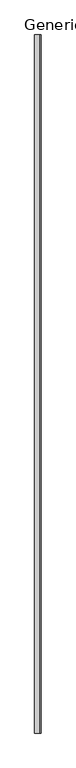
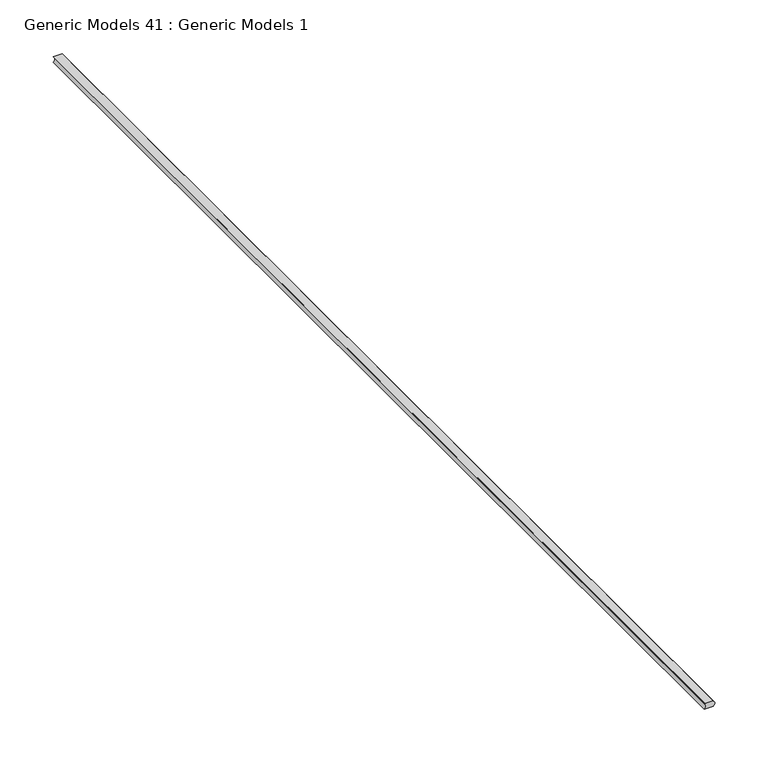
"""IFC4 building model written with IfcOpenShell, lengths in millimetres: proxy geometry, Generic Models 41 : Generic Models 1."""

from ifc_helpers import new_model, si_unit, point, frame, frame_2d, origin, place, context, project, spatial, polyline, circle_curve, trimmed, segment, composite_curve, outline, extrude, source, transform, mapped, element, save


def generic_models_41_generic_models_1_f9918aae(model_context):
    return source(origin(), model_context, "Body", "SweptSolid", [
        extrude(outline(composite_curve([segment(polyline([(0.0, 50777.775), (0.0, 50787.3)]), True, "CONTINUOUS"), segment(trimmed(circle_curve(frame_2d((3.175, 50784.3852595)), 4.3100275), [point((0.0, 50787.3))], [point((6.35, 50787.3))], False, "CARTESIAN"), True, "CONTINUOUS"), segment(polyline([(6.35, 50787.3), (6.35, 50777.775)]), True, "CONTINUOUS"), segment(trimmed(circle_curve(frame_2d((3.175, 50774.8602595)), 4.3100275), [point((6.35, 50777.775))], [point((0.0, 50777.775))], True, "CARTESIAN"), True, "CONTINUOUS")], self_intersect=False)), frame((0.0, 0.0, 0.0), z_axis=(0.0, 1.0, 0.0), x_axis=(0.0, 0.0, 1.0)), (0.0, 0.0, 1.0), 1219.2),
    ])


if __name__ == "__main__":
    model = new_model("IFC4")
    model_context = context("Model", 3, world=origin())
    ifc_project = project(units=[si_unit("LENGTHUNIT", "METRE", prefix="MILLI")], contexts=[model_context])
    site = spatial("IfcSite", under=ifc_project)
    building = spatial("IfcBuilding", under=site)
    placement = place(None, origin())
    generic_models_41_generic_models_1_shape = generic_models_41_generic_models_1_f9918aae(model_context)
    element("IfcBuildingElementProxy", 1, Name="Generic Models 41 : Generic Models 1", ObjectType="Generic Models 41 : Generic Models 1", at=placement, inside=building, context=model_context, shape_type="MappedRepresentation", body=[
        mapped(generic_models_41_generic_models_1_shape, transform((0.0, 0.0, 0.0), x_axis=(1.0, 0.0, 0.0), y_axis=(0.0, 1.0, 0.0), z_axis=(0.0, 0.0, 1.0))),
    ])
    save(model, "model.ifc")

# Revit data of these elements
# Element 1 (IfcBuildingElementProxy, "Generic Models 41 : Generic Models 1")
#   Materials on its faces: "ACOUSTICAL SEALANT"
# Materials
#   "ACOUSTICAL SEALANT": class "Unassigned", colour RGB 120 120 120, transparency 0, Cost = 0
